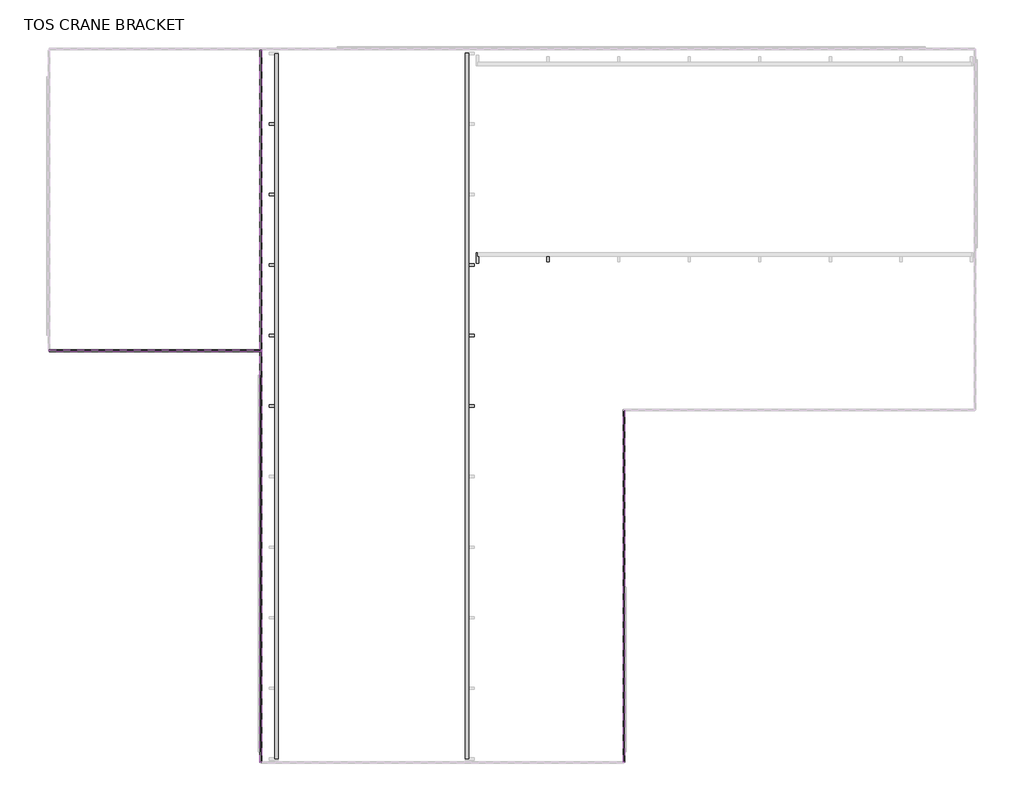
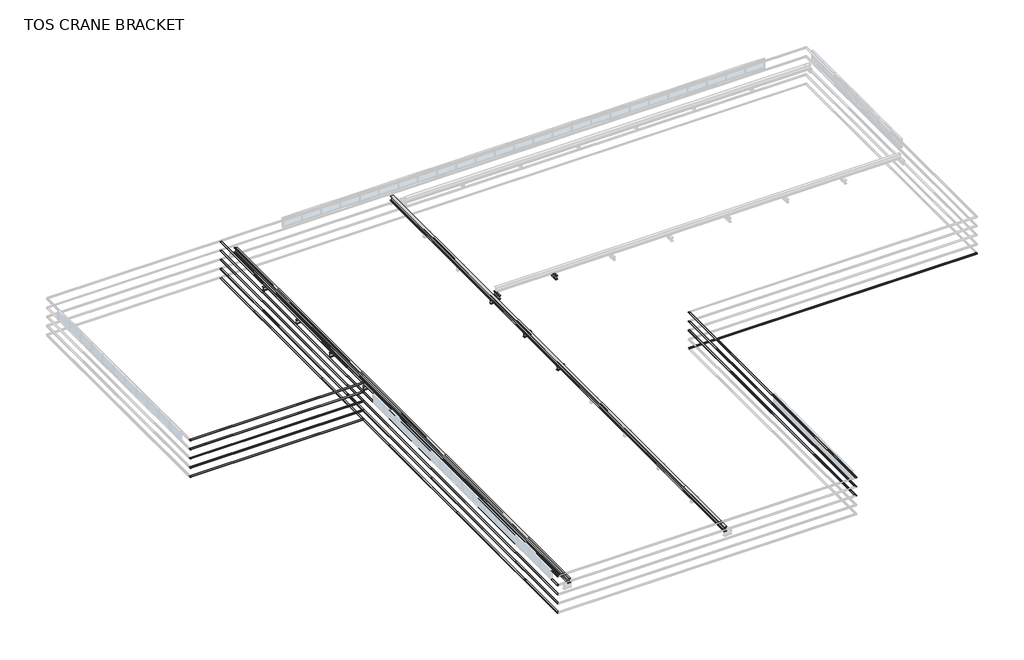
# One storey, part 2 of 3: 26 beams.
"""IFC4 building model written with IfcOpenShell, lengths in millimetres."""

import ifcopenshell
import ifcopenshell.guid

model = None  # the IFC model being written
_history = None  # IfcOwnerHistory: only IFC2X3 demands one
_inside = {}  # id of a spatial element -> (the spatial element, [elements in it])
_under = {}  # id of a project, library or spatial element -> (it, [spatial elements below it])
_declared = {}  # id of a project -> (the project, [libraries it declares])
_typed = {}  # id of a type object -> (the type object, [elements of that type])
_made_of = {}  # id of a material, layer set ... -> (it, [elements and type objects made of it])


def new_model(schema):
    """Start an empty IFC model of exactly this schema.

    Asked for "IFC4X3", IfcOpenShell would pick the latest addendum, in which some entities
    have other attributes; the version numbers below select the first issue.
    IFC2X3 requires an IfcOwnerHistory on every rooted entity: one is made here for all.
    """
    global model, _history
    if schema == "IFC4X3":
        model = ifcopenshell.file(schema_version=(4, 3, 0, 0))
    else:
        model = ifcopenshell.file(schema=schema)
    _inside.clear()
    _under.clear()
    _declared.clear()
    _typed.clear()
    _made_of.clear()
    _history = None
    if model.schema == "IFC2X3":
        org = make("IfcOrganization", Name="unknown")
        user = make(
            "IfcPersonAndOrganization",
            ThePerson=make("IfcPerson", FamilyName="unknown"),
            TheOrganization=org,
        )
        app = make(
            "IfcApplication",
            ApplicationDeveloper=org,
            Version="unknown",
            ApplicationFullName="unknown",
            ApplicationIdentifier="unknown",
        )
        _history = make(
            "IfcOwnerHistory",
            OwningUser=user,
            OwningApplication=app,
            ChangeAction="ADDED",
            CreationDate=0,
        )
    return model


def make(cls, **values):
    """One entity of the class cls with the attributes given. An attribute that is None is left unset."""
    return model.create_entity(
        cls, **{name: value for name, value in values.items() if value is not None}
    )


def rooted(cls, **values):
    """An entity with a GlobalId (a new one), such as an element, a storey or a relation."""
    return make(cls, GlobalId=ifcopenshell.guid.new(), OwnerHistory=_history, **values)


def si_unit(unit_type, name, prefix=None):
    """IfcSIUnit, for example si_unit("LENGTHUNIT", "METRE", prefix="MILLI")."""
    return make("IfcSIUnit", UnitType=unit_type, Prefix=prefix, Name=name)


def assignment(units):
    """IfcUnitAssignment: the units of a project."""
    return None if units is None else make("IfcUnitAssignment", Units=units)


def point(xyz):
    """IfcCartesianPoint."""
    return None if xyz is None else make("IfcCartesianPoint", Coordinates=xyz)


def direction(xyz):
    """IfcDirection."""
    return None if xyz is None else make("IfcDirection", DirectionRatios=xyz)


def frame(location, z_axis=None, x_axis=None):
    """IfcAxis2Placement3D, a coordinate frame: its origin and axes. An axis left out is left unset."""
    return make(
        "IfcAxis2Placement3D",
        Location=point(location),
        Axis=direction(z_axis),
        RefDirection=direction(x_axis),
    )


def frame_2d(location, x_axis=None):
    """IfcAxis2Placement2D, a coordinate frame in the plane: its origin and x axis."""
    return make(
        "IfcAxis2Placement2D", Location=point(location), RefDirection=direction(x_axis)
    )


def origin():
    """The frame at (0, 0, 0) with its axes left unset."""
    return frame((0.0, 0.0, 0.0))


def place(relative_to, where):
    """IfcLocalPlacement: puts the frame where relative to a parent placement (None: the world)."""
    return make(
        "IfcLocalPlacement", PlacementRelTo=relative_to, RelativePlacement=where
    )


def context(
    kind, dimensions, precision=None, world=None, true_north=None, identifier=None
):
    """IfcGeometricRepresentationContext, for example the 3D "Model" context."""
    return make(
        "IfcGeometricRepresentationContext",
        ContextIdentifier=identifier,
        ContextType=kind,
        CoordinateSpaceDimension=dimensions,
        Precision=precision,
        WorldCoordinateSystem=world,
        TrueNorth=true_north,
    )


def project(units=None, contexts=None):
    """IfcProject with its units and contexts."""
    return rooted(
        "IfcProject",
        Name="project",
        RepresentationContexts=contexts,
        UnitsInContext=assignment(units),
    )


def spatial(cls, under=None, at=None, **own):
    """A site, building, storey or space (cls), placed at a placement, below another one or the project."""
    s = rooted(cls, ObjectPlacement=at, **own)
    if under is not None:
        _under.setdefault(under.id(), (under, []))[1].append(s)
    return s


def polyline(points):
    """IfcPolyline through the points."""
    return make("IfcPolyline", Points=[point(p) for p in points])


def circle_curve(where, radius):
    """IfcCircle in the frame where."""
    return make("IfcCircle", Position=where, Radius=radius)


def trimmed(basis, trim1, trim2, sense, master):
    """IfcTrimmedCurve: the piece of a basis curve between two trims."""
    return make(
        "IfcTrimmedCurve",
        BasisCurve=basis,
        Trim1=trim1,
        Trim2=trim2,
        SenseAgreement=sense,
        MasterRepresentation=master,
    )


def segment(curve, same_sense, transition):
    """IfcCompositeCurveSegment."""
    return make(
        "IfcCompositeCurveSegment",
        Transition=transition,
        SameSense=same_sense,
        ParentCurve=curve,
    )


def composite_curve(segments, self_intersect=None):
    """IfcCompositeCurve: segments joined end to end."""
    return make("IfcCompositeCurve", Segments=segments, SelfIntersect=self_intersect)


def outline(outer, holes=None, kind="AREA"):
    """IfcArbitraryClosedProfileDef: a profile drawn as a closed curve; with holes, ...WithVoids."""
    if holes is None:
        return make("IfcArbitraryClosedProfileDef", ProfileType=kind, OuterCurve=outer)
    return make(
        "IfcArbitraryProfileDefWithVoids",
        ProfileType=kind,
        OuterCurve=outer,
        InnerCurves=holes,
    )


def extrude(swept, where, along, depth):
    """IfcExtrudedAreaSolid: the profile swept, set in the frame where, extruded along a direction by depth."""
    return make(
        "IfcExtrudedAreaSolid",
        SweptArea=swept,
        Position=where,
        ExtrudedDirection=direction(along),
        Depth=depth,
    )


def shape(context_of_items, identifier, shape_type, items):
    """IfcShapeRepresentation: the items that make up one representation, for example the "Body"."""
    return make(
        "IfcShapeRepresentation",
        ContextOfItems=context_of_items,
        RepresentationIdentifier=identifier,
        RepresentationType=shape_type,
        Items=items,
    )


def source(mapping_origin, context_of_items, identifier, shape_type, items):
    """IfcRepresentationMap: a shape defined once, which mapped items show again and again."""
    return make(
        "IfcRepresentationMap",
        MappingOrigin=mapping_origin,
        MappedRepresentation=shape(context_of_items, identifier, shape_type, items),
    )


def transform(
    local_origin,
    x_axis=None,
    y_axis=None,
    z_axis=None,
    scale=None,
    scale2=None,
    scale3=None,
    uniform=True,
):
    """IfcCartesianTransformationOperator3D, or its non-uniform kind. x_axis, y_axis, z_axis: its Axis1, 2, 3."""
    if uniform:
        return make(
            "IfcCartesianTransformationOperator3D",
            Axis1=direction(x_axis),
            Axis2=direction(y_axis),
            LocalOrigin=point(local_origin),
            Scale=scale,
            Axis3=direction(z_axis),
        )
    return make(
        "IfcCartesianTransformationOperator3DnonUniform",
        Axis1=direction(x_axis),
        Axis2=direction(y_axis),
        LocalOrigin=point(local_origin),
        Scale=scale,
        Axis3=direction(z_axis),
        Scale2=scale2,
        Scale3=scale3,
    )


def mapped(mapping_source, mapping_target):
    """IfcMappedItem: shows the shape of a source again, moved by a transform."""
    return make(
        "IfcMappedItem", MappingSource=mapping_source, MappingTarget=mapping_target
    )


def made_of(thing, what):
    """Note that an element or type object is made of a material, layer set ...; save() writes the relation."""
    if what is not None:
        _made_of.setdefault(what.id(), (what, []))[1].append(thing)
    return thing


def element(
    cls,
    number,
    at=None,
    inside=None,
    cuts=None,
    type_object=None,
    material=None,
    context=None,
    identifier="Body",
    shape_type=None,
    held_by="IfcProductDefinitionShape",
    body=None,
    shapes=None,
    **own,
):
    """One element of the class cls, such as IfcWall. Its Tag is "e" and its number.

    at: its placement. inside: the storey or other place that contains it. cuts: it is an
    opening in that element (IfcRelVoidsElement). A single representation is given by context,
    identifier, shape_type and body (its items); several are given by shapes. held_by: the class
    of the entity that holds the representations. save() writes the other relations.
    """
    e = rooted(cls, Tag="e%d" % number, ObjectPlacement=at, **own)
    if body is not None:
        shapes = [shape(context, identifier, shape_type, body)]
    if shapes is not None:
        e.Representation = make(held_by, Representations=shapes)
    if inside is not None:
        _inside.setdefault(inside.id(), (inside, []))[1].append(e)
    if cuts is not None:
        rooted(
            "IfcRelVoidsElement", RelatingBuildingElement=cuts, RelatedOpeningElement=e
        )
    if type_object is not None:
        _typed.setdefault(type_object.id(), (type_object, []))[1].append(e)
    return made_of(e, material)


def aggregate(whole, parts):
    """IfcRelAggregates: a whole, such as a stair, and the parts it consists of."""
    return rooted("IfcRelAggregates", RelatingObject=whole, RelatedObjects=parts)


def save(model, path):
    """Write the relations noted so far, then the file.

    IfcRelAggregates (storeys below a building ...), IfcRelContainedInSpatialStructure (elements
    in a storey), IfcRelDefinesByType, IfcRelAssociatesMaterial and IfcRelDeclares: one each for
    every whole, place, type object, material and project.
    """
    for whole, parts in _under.values():
        aggregate(whole, parts)
    for where, things in _inside.values():
        rooted(
            "IfcRelContainedInSpatialStructure",
            RelatedElements=things,
            RelatingStructure=where,
        )
    for kind, things in _typed.values():
        rooted("IfcRelDefinesByType", RelatedObjects=things, RelatingType=kind)
    for what, things in _made_of.values():
        rooted("IfcRelAssociatesMaterial", RelatedObjects=things, RelatingMaterial=what)
    for by, libraries in _declared.values():
        rooted("IfcRelDeclares", RelatingContext=by, RelatedDefinitions=libraries)
    model.write(path)


def beam_70e5a2de(model_context):
    return source(origin(), model_context, "Body", "SweptSolid", [
        extrude(outline(composite_curve([segment(polyline([(150.0, -226.0), (150.0, -244.0), (-150.0, -244.0), (-150.0, -226.0), (-31.5, -226.0)]), True, "CONTINUOUS"), segment(trimmed(circle_curve(frame_2d((-31.5, -200.0)), 26.0), [point((-31.5, -226.0))], [point((-5.5, -200.0))], True, "CARTESIAN"), True, "CONTINUOUS"), segment(polyline([(-5.5, -200.0), (-5.5, 200.0)]), True, "CONTINUOUS"), segment(trimmed(circle_curve(frame_2d((-31.5, 200.0)), 26.0), [point((-5.5, 200.0))], [point((-31.5, 226.0))], True, "CARTESIAN"), True, "CONTINUOUS"), segment(polyline([(-31.5, 226.0), (-150.0, 226.0), (-150.0, 244.0), (150.0, 244.0), (150.0, 226.0), (31.5, 226.0)]), True, "CONTINUOUS"), segment(trimmed(circle_curve(frame_2d((31.5, 200.0)), 26.0), [point((31.5, 226.0))], [point((5.5, 200.0))], True, "CARTESIAN"), True, "CONTINUOUS"), segment(polyline([(5.5, 200.0), (5.5, -200.0)]), True, "CONTINUOUS"), segment(trimmed(circle_curve(frame_2d((31.5, -200.0)), 26.0), [point((5.5, -200.0))], [point((31.5, -226.0))], True, "CARTESIAN"), True, "CONTINUOUS"), segment(polyline([(31.5, -226.0), (150.0, -226.0)]), True, "CONTINUOUS")], self_intersect=False)), frame((-30000.0, 0.0, 0.0), z_axis=(1.0, 0.0, 0.0), x_axis=(0.0, 1.0, 0.0)), (0.0, 0.0, 1.0), 60000.0),
    ])


def beam_a081c7c9(model_context):
    return source(origin(), model_context, "Body", "SweptSolid", [
        extrude(outline(composite_curve([segment(polyline([(100.0, -187.0), (100.0, -200.0), (-100.0, -200.0), (-100.0, -187.0), (-20.0, -187.0)]), True, "CONTINUOUS"), segment(trimmed(circle_curve(frame_2d((-20.0, -171.0)), 16.0), [point((-20.0, -187.0))], [point((-4.0, -171.0))], True, "CARTESIAN"), True, "CONTINUOUS"), segment(polyline([(-4.0, -171.0), (-4.0, 171.0)]), True, "CONTINUOUS"), segment(trimmed(circle_curve(frame_2d((-20.0, 171.0)), 16.0), [point((-4.0, 171.0))], [point((-20.0, 187.0))], True, "CARTESIAN"), True, "CONTINUOUS"), segment(polyline([(-20.0, 187.0), (-100.0, 187.0), (-100.0, 200.0), (100.0, 200.0), (100.0, 187.0), (20.0, 187.0)]), True, "CONTINUOUS"), segment(trimmed(circle_curve(frame_2d((20.0, 171.0)), 16.0), [point((20.0, 187.0))], [point((4.0, 171.0))], True, "CARTESIAN"), True, "CONTINUOUS"), segment(polyline([(4.0, 171.0), (4.0, -171.0)]), True, "CONTINUOUS"), segment(trimmed(circle_curve(frame_2d((20.0, -171.0)), 16.0), [point((4.0, -171.0))], [point((20.0, -187.0))], True, "CARTESIAN"), True, "CONTINUOUS"), segment(polyline([(20.0, -187.0), (100.0, -187.0)]), True, "CONTINUOUS")], self_intersect=False)), frame((-236.0, 0.0, 0.0), z_axis=(1.0, 0.0, 0.0), x_axis=(0.0, 1.0, 0.0)), (0.0, 0.0, 1.0), 766.0),
    ])


def beam_d36fe593(model_context):
    return source(origin(), model_context, "Body", "SweptSolid", [
        extrude(outline(composite_curve([segment(polyline([(-100.0, -187.0), (-20.0, -187.0)]), True, "CONTINUOUS"), segment(trimmed(circle_curve(frame_2d((-20.0, -171.0)), 16.0), [point((-20.0, -187.0))], [point((-4.0, -171.0))], True, "CARTESIAN"), True, "CONTINUOUS"), segment(polyline([(-4.0, -171.0), (-4.0, 171.0)]), True, "CONTINUOUS"), segment(trimmed(circle_curve(frame_2d((-20.0, 171.0)), 16.0), [point((-4.0, 171.0))], [point((-20.0, 187.0))], True, "CARTESIAN"), True, "CONTINUOUS"), segment(polyline([(-20.0, 187.0), (-100.0, 187.0), (-100.0, 200.0), (100.0, 200.0), (100.0, 187.0), (20.0, 187.0)]), True, "CONTINUOUS"), segment(trimmed(circle_curve(frame_2d((20.0, 171.0)), 16.0), [point((20.0, 187.0))], [point((4.0, 171.0))], True, "CARTESIAN"), True, "CONTINUOUS"), segment(polyline([(4.0, 171.0), (4.0, -171.0)]), True, "CONTINUOUS"), segment(trimmed(circle_curve(frame_2d((20.0, -171.0)), 16.0), [point((4.0, -171.0))], [point((20.0, -187.0))], True, "CARTESIAN"), True, "CONTINUOUS"), segment(polyline([(20.0, -187.0), (100.0, -187.0), (100.0, -200.0), (-100.0, -200.0), (-100.0, -187.0)]), True, "CONTINUOUS")], self_intersect=False)), frame((-236.0, 0.0, 0.0), z_axis=(1.0, 0.0, 0.0), x_axis=(0.0, 1.0, 0.0)), (0.0, 0.0, 1.0), 766.0),
    ])


def beam_06871935(model_context):
    return source(origin(), model_context, "Body", "SweptSolid", [
        extrude(outline(composite_curve([segment(polyline([(-150.0, -226.0), (-31.5, -226.0)]), True, "CONTINUOUS"), segment(trimmed(circle_curve(frame_2d((-31.5, -200.0)), 26.0), [point((-31.5, -226.0))], [point((-5.5, -200.0))], True, "CARTESIAN"), True, "CONTINUOUS"), segment(polyline([(-5.5, -200.0), (-5.5, 200.0)]), True, "CONTINUOUS"), segment(trimmed(circle_curve(frame_2d((-31.5, 200.0)), 26.0), [point((-5.5, 200.0))], [point((-31.5, 226.0))], True, "CARTESIAN"), True, "CONTINUOUS"), segment(polyline([(-31.5, 226.0), (-150.0, 226.0), (-150.0, 244.0), (150.0, 244.0), (150.0, 226.0), (31.5, 226.0)]), True, "CONTINUOUS"), segment(trimmed(circle_curve(frame_2d((31.5, 200.0)), 26.0), [point((31.5, 226.0))], [point((5.5, 200.0))], True, "CARTESIAN"), True, "CONTINUOUS"), segment(polyline([(5.5, 200.0), (5.5, -200.0)]), True, "CONTINUOUS"), segment(trimmed(circle_curve(frame_2d((31.5, -200.0)), 26.0), [point((5.5, -200.0))], [point((31.5, -226.0))], True, "CARTESIAN"), True, "CONTINUOUS"), segment(polyline([(31.5, -226.0), (150.0, -226.0), (150.0, -244.0), (-150.0, -244.0), (-150.0, -226.0)]), True, "CONTINUOUS")], self_intersect=False)), frame((-29987.2, 0.0, 0.0), z_axis=(1.0, 0.0, 0.0), x_axis=(0.0, 1.0, 0.0)), (0.0, 0.0, 1.0), 59974.4),
    ])


def beam_29f4eb64(model_context):
    return source(origin(), model_context, "Body", "SweptSolid", [
        extrude(outline(composite_curve([segment(polyline([(-100.0, -187.0), (-20.0, -187.0)]), True, "CONTINUOUS"), segment(trimmed(circle_curve(frame_2d((-20.0, -171.0)), 16.0), [point((-20.0, -187.0))], [point((-4.0, -171.0))], True, "CARTESIAN"), True, "CONTINUOUS"), segment(polyline([(-4.0, -171.0), (-4.0, 171.0)]), True, "CONTINUOUS"), segment(trimmed(circle_curve(frame_2d((-20.0, 171.0)), 16.0), [point((-4.0, 171.0))], [point((-20.0, 187.0))], True, "CARTESIAN"), True, "CONTINUOUS"), segment(polyline([(-20.0, 187.0), (-100.0, 187.0), (-100.0, 200.0), (100.0, 200.0), (100.0, 187.0), (20.0, 187.0)]), True, "CONTINUOUS"), segment(trimmed(circle_curve(frame_2d((20.0, 171.0)), 16.0), [point((20.0, 187.0))], [point((4.0, 171.0))], True, "CARTESIAN"), True, "CONTINUOUS"), segment(polyline([(4.0, 171.0), (4.0, -171.0)]), True, "CONTINUOUS"), segment(trimmed(circle_curve(frame_2d((20.0, -171.0)), 16.0), [point((4.0, -171.0))], [point((20.0, -187.0))], True, "CARTESIAN"), True, "CONTINUOUS"), segment(polyline([(20.0, -187.0), (100.0, -187.0), (100.0, -200.0), (-100.0, -200.0), (-100.0, -187.0)]), True, "CONTINUOUS")], self_intersect=False)), frame((-380.0, 0.0, 0.0), z_axis=(1.0, 0.0, 0.0), x_axis=(0.0, 1.0, 0.0)), (0.0, 0.0, 1.0), 910.0),
    ])


def steel_framing_lc_58cf0942(model_context):
    return source(origin(), model_context, "Body", "SweptSolid", [
        extrude(outline(composite_curve([segment(polyline([(18.6, 67.0), (18.6, -67.0)]), True, "CONTINUOUS"), segment(trimmed(circle_curve(frame_2d((10.6, -67.0)), 8.0), [point((18.6, -67.0))], [point((10.6, -75.0))], False, "CARTESIAN"), True, "CONTINUOUS"), segment(polyline([(10.6, -75.0), (-48.4, -75.0)]), True, "CONTINUOUS"), segment(trimmed(circle_curve(frame_2d((-48.4, -67.0)), 8.0), [point((-48.4, -75.0))], [point((-56.4, -67.0))], False, "CARTESIAN"), True, "CONTINUOUS"), segment(polyline([(-56.4, -67.0), (-56.4, -50.0), (-53.2, -50.0), (-53.2, -67.0)]), True, "CONTINUOUS"), segment(trimmed(circle_curve(frame_2d((-48.4, -67.0)), 4.8), [point((-53.2, -67.0))], [point((-48.4, -71.8))], True, "CARTESIAN"), True, "CONTINUOUS"), segment(polyline([(-48.4, -71.8), (10.6, -71.8)]), True, "CONTINUOUS"), segment(trimmed(circle_curve(frame_2d((10.6, -67.0)), 4.8), [point((10.6, -71.8))], [point((15.4, -67.0))], True, "CARTESIAN"), True, "CONTINUOUS"), segment(polyline([(15.4, -67.0), (15.4, 67.0)]), True, "CONTINUOUS"), segment(trimmed(circle_curve(frame_2d((10.6, 67.0)), 4.8), [point((15.4, 67.0))], [point((10.6, 71.8))], True, "CARTESIAN"), True, "CONTINUOUS"), segment(polyline([(10.6, 71.8), (-48.4, 71.8)]), True, "CONTINUOUS"), segment(trimmed(circle_curve(frame_2d((-48.4, 67.0)), 4.8), [point((-48.4, 71.8))], [point((-53.2, 67.0))], True, "CARTESIAN"), True, "CONTINUOUS"), segment(polyline([(-53.2, 67.0), (-53.2, 50.0), (-56.4, 50.0), (-56.4, 67.0)]), True, "CONTINUOUS"), segment(trimmed(circle_curve(frame_2d((-48.4, 67.0)), 8.0), [point((-56.4, 67.0))], [point((-48.4, 75.0))], False, "CARTESIAN"), True, "CONTINUOUS"), segment(polyline([(-48.4, 75.0), (10.6, 75.0)]), True, "CONTINUOUS"), segment(trimmed(circle_curve(frame_2d((10.6, 67.0)), 8.0), [point((10.6, 75.0))], [point((18.6, 67.0))], False, "CARTESIAN"), True, "CONTINUOUS")], self_intersect=False)), frame((-30297.0, 0.0, 0.0), z_axis=(1.0, 0.0, 0.0), x_axis=(0.0, 1.0, 0.0)), (0.0, 0.0, 1.0), 60581.0),
    ])


model = new_model("IFC4")

# Units and contexts
model_context = context("Model", 3, world=origin())
ifc_project = project(units=[si_unit("LENGTHUNIT", "METRE", prefix="MILLI")], contexts=[model_context])

# Site, building, storey
site = spatial("IfcSite", under=ifc_project)
building = spatial("IfcBuilding", under=site)
storey = spatial("IfcBuildingStorey", under=building, Name="TOS CRANE BRACKET", Elevation=6699.9618634)

# Beams
placement = place(None, origin())
beam_shape = beam_70e5a2de(model_context)
element("IfcBeam", 1, ObjectType="Steel Framing_H_KS : H_SB_AR_S02_H-488x300x11x18_CRG1", at=placement, inside=storey, context=model_context, shape_type="MappedRepresentation", body=[
    mapped(beam_shape, transform((35100.0, -30000.0, 6953.9618634), x_axis=(0.0, 1.0, 0.0), y_axis=(-1.0, 0.0, 0.0), z_axis=(0.0, 0.0, 1.0))),
])
beam_2_shape = beam_a081c7c9(model_context)
element("IfcBeam", 2, ObjectType="Steel Framing_H_KS : H_SB_AR_S02_H-400x200x8x13_SCB1", at=placement, inside=storey, context=model_context, shape_type="MappedRepresentation", body=[
    mapped(beam_2_shape, transform((35470.0, -18000.0, 6499.9618634), x_axis=(-1.0, 0.0, 0.0), y_axis=(0.0, -1.0, 0.0), z_axis=(0.0, 0.0, 1.0))),
])
element("IfcBeam", 3, ObjectType="Steel Framing_H_KS : H_SB_AR_S02_H-400x200x8x13_SCB1", at=placement, inside=storey, context=model_context, shape_type="MappedRepresentation", body=[
    mapped(beam_2_shape, transform((35470.0, -24000.0, 6499.9618634), x_axis=(-1.0, 0.0, 0.0), y_axis=(0.0, -1.0, 0.0), z_axis=(0.0, 0.0, 1.0))),
])
element("IfcBeam", 4, ObjectType="Steel Framing_H_KS : H_SB_AR_S02_H-400x200x8x13_SCB1", at=placement, inside=storey, context=model_context, shape_type="MappedRepresentation", body=[
    mapped(beam_2_shape, transform((35470.0, -30000.0, 6499.9618634), x_axis=(-1.0, 0.0, 0.0), y_axis=(0.0, -1.0, 0.0), z_axis=(0.0, 0.0, 1.0))),
])
beam_3_shape = beam_d36fe593(model_context)
element("IfcBeam", 5, ObjectType="Steel Framing_H_KS : H_SB_AR_S02_H-400x200x8x13_SCB1", at=placement, inside=storey, context=model_context, shape_type="MappedRepresentation", body=[
    mapped(beam_3_shape, transform((18530.0, -6000.0, 6499.9618634), x_axis=(1.0, 0.0, 0.0), y_axis=(0.0, 1.0, 0.0), z_axis=(0.0, 0.0, 1.0))),
])
element("IfcBeam", 6, ObjectType="Steel Framing_H_KS : H_SB_AR_S02_H-400x200x8x13_SCB1", at=placement, inside=storey, context=model_context, shape_type="MappedRepresentation", body=[
    mapped(beam_3_shape, transform((18530.0, -12000.0, 6499.9618634), x_axis=(1.0, 0.0, 0.0), y_axis=(0.0, 1.0, 0.0), z_axis=(0.0, 0.0, 1.0))),
])
element("IfcBeam", 7, ObjectType="Steel Framing_H_KS : H_SB_AR_S02_H-400x200x8x13_SCB1", at=placement, inside=storey, context=model_context, shape_type="MappedRepresentation", body=[
    mapped(beam_3_shape, transform((18530.0, -18000.0, 6499.9618634), x_axis=(1.0, 0.0, 0.0), y_axis=(0.0, 1.0, 0.0), z_axis=(0.0, 0.0, 1.0))),
])
element("IfcBeam", 8, ObjectType="Steel Framing_H_KS : H_SB_AR_S02_H-400x200x8x13_SCB1", at=placement, inside=storey, context=model_context, shape_type="MappedRepresentation", body=[
    mapped(beam_3_shape, transform((18530.0, -24000.0, 6499.9618634), x_axis=(1.0, 0.0, 0.0), y_axis=(0.0, 1.0, 0.0), z_axis=(0.0, 0.0, 1.0))),
])
element("IfcBeam", 9, ObjectType="Steel Framing_H_KS : H_SB_AR_S02_H-400x200x8x13_SCB1", at=placement, inside=storey, context=model_context, shape_type="MappedRepresentation", body=[
    mapped(beam_3_shape, transform((18530.0, -30000.0, 6499.9618634), x_axis=(1.0, 0.0, 0.0), y_axis=(0.0, 1.0, 0.0), z_axis=(0.0, 0.0, 1.0))),
])
element("IfcBeam", 10, ObjectType="Steel Framing_H_KS : H_SB_AR_S02_H-400x200x8x13_SCB1", at=placement, inside=storey, context=model_context, shape_type="MappedRepresentation", body=[
    mapped(beam_3_shape, transform((42000.0, -17470.0, 6499.9618634), x_axis=(0.0, 1.0, 0.0), y_axis=(-1.0, 0.0, 0.0), z_axis=(0.0, 0.0, 1.0))),
])
beam_4_shape = beam_06871935(model_context)
element("IfcBeam", 11, ObjectType="Steel Framing_H_KS : H_SB_AR_S02_H-488x300x11x18_CRG1", at=placement, inside=storey, context=model_context, shape_type="MappedRepresentation", body=[
    mapped(beam_4_shape, transform((18900.0, -30000.0, 6953.9618634), x_axis=(0.0, 1.0, 0.0), y_axis=(-1.0, 0.0, 0.0), z_axis=(0.0, 0.0, 1.0))),
])
beam_5_shape = beam_29f4eb64(model_context)
element("IfcBeam", 12, ObjectType="Steel Framing_H_KS : H_SB_AR_S02_H-400x200x8x13_SCB1", at=placement, inside=storey, context=model_context, shape_type="MappedRepresentation", body=[
    mapped(beam_5_shape, transform((36000.0, -17470.0, 6499.9618634), x_axis=(0.0, 1.0, 0.0), y_axis=(-1.0, 0.0, 0.0), z_axis=(0.0, 0.0, 1.0))),
])
element("IfcBeam", 13, ObjectType="Steel Framing_LC : H_SB_AR_S00_LC-150x75x25x3.2", at=placement, inside=storey, context=model_context, shape_type="SweptSolid", body=[
    extrude(outline(composite_curve([segment(trimmed(circle_curve(frame_2d((-25233.0, 4160.5618634)), 8.0), [point((-25233.0, 4168.5618634))], [point((-25225.0, 4160.5618634))], False, "CARTESIAN"), True, "CONTINUOUS"), segment(polyline([(-25225.0, 4160.5618634), (-25225.0, 4101.5618634)]), True, "CONTINUOUS"), segment(trimmed(circle_curve(frame_2d((-25233.0, 4101.5618634)), 8.0), [point((-25225.0, 4101.5618634))], [point((-25233.0, 4093.5618634))], False, "CARTESIAN"), True, "CONTINUOUS"), segment(polyline([(-25233.0, 4093.5618634), (-25250.0, 4093.5618634), (-25250.0, 4096.7618634), (-25233.0, 4096.7618634)]), True, "CONTINUOUS"), segment(trimmed(circle_curve(frame_2d((-25233.0, 4101.5618634)), 4.8), [point((-25233.0, 4096.7618634))], [point((-25228.2, 4101.5618634))], True, "CARTESIAN"), True, "CONTINUOUS"), segment(polyline([(-25228.2, 4101.5618634), (-25228.2, 4160.5618634)]), True, "CONTINUOUS"), segment(trimmed(circle_curve(frame_2d((-25233.0, 4160.5618634)), 4.8), [point((-25228.2, 4160.5618634))], [point((-25233.0, 4165.3618634))], True, "CARTESIAN"), True, "CONTINUOUS"), segment(polyline([(-25233.0, 4165.3618634), (-25367.0, 4165.3618634)]), True, "CONTINUOUS"), segment(trimmed(circle_curve(frame_2d((-25367.0, 4160.5618634)), 4.8), [point((-25367.0, 4165.3618634))], [point((-25371.8, 4160.5618634))], True, "CARTESIAN"), True, "CONTINUOUS"), segment(polyline([(-25371.8, 4160.5618634), (-25371.8, 4101.5618634)]), True, "CONTINUOUS"), segment(trimmed(circle_curve(frame_2d((-25367.0, 4101.5618634)), 4.8), [point((-25371.8, 4101.5618634))], [point((-25367.0, 4096.7618634))], True, "CARTESIAN"), True, "CONTINUOUS"), segment(polyline([(-25367.0, 4096.7618634), (-25350.0, 4096.7618634), (-25350.0, 4093.5618634), (-25367.0, 4093.5618634)]), True, "CONTINUOUS"), segment(trimmed(circle_curve(frame_2d((-25367.0, 4101.5618634)), 8.0), [point((-25367.0, 4093.5618634))], [point((-25375.0, 4101.5618634))], False, "CARTESIAN"), True, "CONTINUOUS"), segment(polyline([(-25375.0, 4101.5618634), (-25375.0, 4160.5618634)]), True, "CONTINUOUS"), segment(trimmed(circle_curve(frame_2d((-25367.0, 4160.5618634)), 8.0), [point((-25375.0, 4160.5618634))], [point((-25367.0, 4168.5618634))], False, "CARTESIAN"), True, "CONTINUOUS"), segment(polyline([(-25367.0, 4168.5618634), (-25233.0, 4168.5618634)]), True, "CONTINUOUS")], self_intersect=False)), frame((-450.0, 0.0, 0.0), z_axis=(1.0, 0.0, 0.0), x_axis=(0.0, 1.0, 0.0)), (0.0, 0.0, 1.0), 18000.0),
])
element("IfcBeam", 14, ObjectType="Steel Framing_LC : H_SB_AR_S00_LC-150x75x25x3.2", at=placement, inside=storey, context=model_context, shape_type="SweptSolid", body=[
    extrude(outline(composite_curve([segment(polyline([(-30392.0, 4168.5618634), (-30258.0, 4168.5618634)]), True, "CONTINUOUS"), segment(trimmed(circle_curve(frame_2d((-30258.0, 4160.5618634)), 8.0), [point((-30258.0, 4168.5618634))], [point((-30250.0, 4160.5618634))], False, "CARTESIAN"), True, "CONTINUOUS"), segment(polyline([(-30250.0, 4160.5618634), (-30250.0, 4101.5618634)]), True, "CONTINUOUS"), segment(trimmed(circle_curve(frame_2d((-30258.0, 4101.5618634)), 8.0), [point((-30250.0, 4101.5618634))], [point((-30258.0, 4093.5618634))], False, "CARTESIAN"), True, "CONTINUOUS"), segment(polyline([(-30258.0, 4093.5618634), (-30275.0, 4093.5618634), (-30275.0, 4096.7618634), (-30258.0, 4096.7618634)]), True, "CONTINUOUS"), segment(trimmed(circle_curve(frame_2d((-30258.0, 4101.5618634)), 4.8), [point((-30258.0, 4096.7618634))], [point((-30253.2, 4101.5618634))], True, "CARTESIAN"), True, "CONTINUOUS"), segment(polyline([(-30253.2, 4101.5618634), (-30253.2, 4160.5618634)]), True, "CONTINUOUS"), segment(trimmed(circle_curve(frame_2d((-30258.0, 4160.5618634)), 4.8), [point((-30253.2, 4160.5618634))], [point((-30258.0, 4165.3618634))], True, "CARTESIAN"), True, "CONTINUOUS"), segment(polyline([(-30258.0, 4165.3618634), (-30392.0, 4165.3618634)]), True, "CONTINUOUS"), segment(trimmed(circle_curve(frame_2d((-30392.0, 4160.5618634)), 4.8), [point((-30392.0, 4165.3618634))], [point((-30396.8, 4160.5618634))], True, "CARTESIAN"), True, "CONTINUOUS"), segment(polyline([(-30396.8, 4160.5618634), (-30396.8, 4101.5618634)]), True, "CONTINUOUS"), segment(trimmed(circle_curve(frame_2d((-30392.0, 4101.5618634)), 4.8), [point((-30396.8, 4101.5618634))], [point((-30392.0, 4096.7618634))], True, "CARTESIAN"), True, "CONTINUOUS"), segment(polyline([(-30392.0, 4096.7618634), (-30375.0, 4096.7618634), (-30375.0, 4093.5618634), (-30392.0, 4093.5618634)]), True, "CONTINUOUS"), segment(trimmed(circle_curve(frame_2d((-30392.0, 4101.5618634)), 8.0), [point((-30392.0, 4093.5618634))], [point((-30400.0, 4101.5618634))], False, "CARTESIAN"), True, "CONTINUOUS"), segment(polyline([(-30400.0, 4101.5618634), (-30400.0, 4160.5618634)]), True, "CONTINUOUS"), segment(trimmed(circle_curve(frame_2d((-30392.0, 4160.5618634)), 8.0), [point((-30400.0, 4160.5618634))], [point((-30392.0, 4168.5618634))], False, "CARTESIAN"), True, "CONTINUOUS")], self_intersect=False)), frame((48450.0, 0.0, 0.0), z_axis=(1.0, 0.0, 0.0), x_axis=(0.0, 1.0, 0.0)), (0.0, 0.0, 1.0), 29850.0),
])
element("IfcBeam", 15, ObjectType="Steel Framing_LC : H_SB_AR_S00_LC-150x75x25x3.2", at=placement, inside=storey, context=model_context, shape_type="SweptSolid", body=[
    extrude(outline(composite_curve([segment(trimmed(circle_curve(frame_2d((-25233.0, 5160.5618634)), 8.0), [point((-25233.0, 5168.5618634))], [point((-25225.0, 5160.5618634))], False, "CARTESIAN"), True, "CONTINUOUS"), segment(polyline([(-25225.0, 5160.5618634), (-25225.0, 5101.5618634)]), True, "CONTINUOUS"), segment(trimmed(circle_curve(frame_2d((-25233.0, 5101.5618634)), 8.0), [point((-25225.0, 5101.5618634))], [point((-25233.0, 5093.5618634))], False, "CARTESIAN"), True, "CONTINUOUS"), segment(polyline([(-25233.0, 5093.5618634), (-25250.0, 5093.5618634), (-25250.0, 5096.7618634), (-25233.0, 5096.7618634)]), True, "CONTINUOUS"), segment(trimmed(circle_curve(frame_2d((-25233.0, 5101.5618634)), 4.8), [point((-25233.0, 5096.7618634))], [point((-25228.2, 5101.5618634))], True, "CARTESIAN"), True, "CONTINUOUS"), segment(polyline([(-25228.2, 5101.5618634), (-25228.2, 5160.5618634)]), True, "CONTINUOUS"), segment(trimmed(circle_curve(frame_2d((-25233.0, 5160.5618634)), 4.8), [point((-25228.2, 5160.5618634))], [point((-25233.0, 5165.3618634))], True, "CARTESIAN"), True, "CONTINUOUS"), segment(polyline([(-25233.0, 5165.3618634), (-25367.0, 5165.3618634)]), True, "CONTINUOUS"), segment(trimmed(circle_curve(frame_2d((-25367.0, 5160.5618634)), 4.8), [point((-25367.0, 5165.3618634))], [point((-25371.8, 5160.5618634))], True, "CARTESIAN"), True, "CONTINUOUS"), segment(polyline([(-25371.8, 5160.5618634), (-25371.8, 5101.5618634)]), True, "CONTINUOUS"), segment(trimmed(circle_curve(frame_2d((-25367.0, 5101.5618634)), 4.8), [point((-25371.8, 5101.5618634))], [point((-25367.0, 5096.7618634))], True, "CARTESIAN"), True, "CONTINUOUS"), segment(polyline([(-25367.0, 5096.7618634), (-25350.0, 5096.7618634), (-25350.0, 5093.5618634), (-25367.0, 5093.5618634)]), True, "CONTINUOUS"), segment(trimmed(circle_curve(frame_2d((-25367.0, 5101.5618634)), 8.0), [point((-25367.0, 5093.5618634))], [point((-25375.0, 5101.5618634))], False, "CARTESIAN"), True, "CONTINUOUS"), segment(polyline([(-25375.0, 5101.5618634), (-25375.0, 5160.5618634)]), True, "CONTINUOUS"), segment(trimmed(circle_curve(frame_2d((-25367.0, 5160.5618634)), 8.0), [point((-25375.0, 5160.5618634))], [point((-25367.0, 5168.5618634))], False, "CARTESIAN"), True, "CONTINUOUS"), segment(polyline([(-25367.0, 5168.5618634), (-25233.0, 5168.5618634)]), True, "CONTINUOUS")], self_intersect=False)), frame((-450.0, 0.0, 0.0), z_axis=(1.0, 0.0, 0.0), x_axis=(0.0, 1.0, 0.0)), (0.0, 0.0, 1.0), 18000.0),
])
element("IfcBeam", 16, ObjectType="Steel Framing_LC : H_SB_AR_S00_LC-150x75x25x3.2", at=placement, inside=storey, context=model_context, shape_type="SweptSolid", body=[
    extrude(outline(composite_curve([segment(trimmed(circle_curve(frame_2d((-25233.0, 6160.5618634)), 8.0), [point((-25233.0, 6168.5618634))], [point((-25225.0, 6160.5618634))], False, "CARTESIAN"), True, "CONTINUOUS"), segment(polyline([(-25225.0, 6160.5618634), (-25225.0, 6101.5618634)]), True, "CONTINUOUS"), segment(trimmed(circle_curve(frame_2d((-25233.0, 6101.5618634)), 8.0), [point((-25225.0, 6101.5618634))], [point((-25233.0, 6093.5618634))], False, "CARTESIAN"), True, "CONTINUOUS"), segment(polyline([(-25233.0, 6093.5618634), (-25250.0, 6093.5618634), (-25250.0, 6096.7618634), (-25233.0, 6096.7618634)]), True, "CONTINUOUS"), segment(trimmed(circle_curve(frame_2d((-25233.0, 6101.5618634)), 4.8), [point((-25233.0, 6096.7618634))], [point((-25228.2, 6101.5618634))], True, "CARTESIAN"), True, "CONTINUOUS"), segment(polyline([(-25228.2, 6101.5618634), (-25228.2, 6160.5618634)]), True, "CONTINUOUS"), segment(trimmed(circle_curve(frame_2d((-25233.0, 6160.5618634)), 4.8), [point((-25228.2, 6160.5618634))], [point((-25233.0, 6165.3618634))], True, "CARTESIAN"), True, "CONTINUOUS"), segment(polyline([(-25233.0, 6165.3618634), (-25367.0, 6165.3618634)]), True, "CONTINUOUS"), segment(trimmed(circle_curve(frame_2d((-25367.0, 6160.5618634)), 4.8), [point((-25367.0, 6165.3618634))], [point((-25371.8, 6160.5618634))], True, "CARTESIAN"), True, "CONTINUOUS"), segment(polyline([(-25371.8, 6160.5618634), (-25371.8, 6101.5618634)]), True, "CONTINUOUS"), segment(trimmed(circle_curve(frame_2d((-25367.0, 6101.5618634)), 4.8), [point((-25371.8, 6101.5618634))], [point((-25367.0, 6096.7618634))], True, "CARTESIAN"), True, "CONTINUOUS"), segment(polyline([(-25367.0, 6096.7618634), (-25350.0, 6096.7618634), (-25350.0, 6093.5618634), (-25367.0, 6093.5618634)]), True, "CONTINUOUS"), segment(trimmed(circle_curve(frame_2d((-25367.0, 6101.5618634)), 8.0), [point((-25367.0, 6093.5618634))], [point((-25375.0, 6101.5618634))], False, "CARTESIAN"), True, "CONTINUOUS"), segment(polyline([(-25375.0, 6101.5618634), (-25375.0, 6160.5618634)]), True, "CONTINUOUS"), segment(trimmed(circle_curve(frame_2d((-25367.0, 6160.5618634)), 8.0), [point((-25375.0, 6160.5618634))], [point((-25367.0, 6168.5618634))], False, "CARTESIAN"), True, "CONTINUOUS"), segment(polyline([(-25367.0, 6168.5618634), (-25233.0, 6168.5618634)]), True, "CONTINUOUS")], self_intersect=False)), frame((-450.0, 0.0, 0.0), z_axis=(1.0, 0.0, 0.0), x_axis=(0.0, 1.0, 0.0)), (0.0, 0.0, 1.0), 18000.0),
])
element("IfcBeam", 17, ObjectType="Steel Framing_LC : H_SB_AR_S00_LC-150x75x25x3.2", at=placement, inside=storey, context=model_context, shape_type="SweptSolid", body=[
    extrude(outline(composite_curve([segment(polyline([(6168.5618634, 48517.0), (6168.5618634, 48383.0)]), True, "CONTINUOUS"), segment(trimmed(circle_curve(frame_2d((6160.5618634, 48383.0)), 8.0), [point((6168.5618634, 48383.0))], [point((6160.5618634, 48375.0))], False, "CARTESIAN"), True, "CONTINUOUS"), segment(polyline([(6160.5618634, 48375.0), (6101.5618634, 48375.0)]), True, "CONTINUOUS"), segment(trimmed(circle_curve(frame_2d((6101.5618634, 48383.0)), 8.0), [point((6101.5618634, 48375.0))], [point((6093.5618634, 48383.0))], False, "CARTESIAN"), True, "CONTINUOUS"), segment(polyline([(6093.5618634, 48383.0), (6093.5618634, 48400.0), (6096.7618634, 48400.0), (6096.7618634, 48383.0)]), True, "CONTINUOUS"), segment(trimmed(circle_curve(frame_2d((6101.5618634, 48383.0)), 4.8), [point((6096.7618634, 48383.0))], [point((6101.5618634, 48378.2))], True, "CARTESIAN"), True, "CONTINUOUS"), segment(polyline([(6101.5618634, 48378.2), (6160.5618634, 48378.2)]), True, "CONTINUOUS"), segment(trimmed(circle_curve(frame_2d((6160.5618634, 48383.0)), 4.8), [point((6160.5618634, 48378.2))], [point((6165.3618634, 48383.0))], True, "CARTESIAN"), True, "CONTINUOUS"), segment(polyline([(6165.3618634, 48383.0), (6165.3618634, 48517.0)]), True, "CONTINUOUS"), segment(trimmed(circle_curve(frame_2d((6160.5618634, 48517.0)), 4.8), [point((6165.3618634, 48517.0))], [point((6160.5618634, 48521.8))], True, "CARTESIAN"), True, "CONTINUOUS"), segment(polyline([(6160.5618634, 48521.8), (6101.5618634, 48521.8)]), True, "CONTINUOUS"), segment(trimmed(circle_curve(frame_2d((6101.5618634, 48517.0)), 4.8), [point((6101.5618634, 48521.8))], [point((6096.7618634, 48517.0))], True, "CARTESIAN"), True, "CONTINUOUS"), segment(polyline([(6096.7618634, 48517.0), (6096.7618634, 48500.0), (6093.5618634, 48500.0), (6093.5618634, 48517.0)]), True, "CONTINUOUS"), segment(trimmed(circle_curve(frame_2d((6101.5618634, 48517.0)), 8.0), [point((6093.5618634, 48517.0))], [point((6101.5618634, 48525.0))], False, "CARTESIAN"), True, "CONTINUOUS"), segment(polyline([(6101.5618634, 48525.0), (6160.5618634, 48525.0)]), True, "CONTINUOUS"), segment(trimmed(circle_curve(frame_2d((6160.5618634, 48517.0)), 8.0), [point((6160.5618634, 48525.0))], [point((6168.5618634, 48517.0))], False, "CARTESIAN"), True, "CONTINUOUS")], self_intersect=False)), frame((0.0, -60300.0, 0.0), z_axis=(0.0, 1.0, 0.0), x_axis=(0.0, 0.0, 1.0)), (0.0, 0.0, 1.0), 29975.0),
])
element("IfcBeam", 18, ObjectType="Steel Framing_LC : H_SB_AR_S00_LC-150x75x25x3.2", at=placement, inside=storey, context=model_context, shape_type="SweptSolid", body=[
    extrude(outline(composite_curve([segment(trimmed(circle_curve(frame_2d((-25233.0, 7160.5618634)), 8.0), [point((-25233.0, 7168.5618634))], [point((-25225.0, 7160.5618634))], False, "CARTESIAN"), True, "CONTINUOUS"), segment(polyline([(-25225.0, 7160.5618634), (-25225.0, 7101.5618634)]), True, "CONTINUOUS"), segment(trimmed(circle_curve(frame_2d((-25233.0, 7101.5618634)), 8.0), [point((-25225.0, 7101.5618634))], [point((-25233.0, 7093.5618634))], False, "CARTESIAN"), True, "CONTINUOUS"), segment(polyline([(-25233.0, 7093.5618634), (-25250.0, 7093.5618634), (-25250.0, 7096.7618634), (-25233.0, 7096.7618634)]), True, "CONTINUOUS"), segment(trimmed(circle_curve(frame_2d((-25233.0, 7101.5618634)), 4.8), [point((-25233.0, 7096.7618634))], [point((-25228.2, 7101.5618634))], True, "CARTESIAN"), True, "CONTINUOUS"), segment(polyline([(-25228.2, 7101.5618634), (-25228.2, 7160.5618634)]), True, "CONTINUOUS"), segment(trimmed(circle_curve(frame_2d((-25233.0, 7160.5618634)), 4.8), [point((-25228.2, 7160.5618634))], [point((-25233.0, 7165.3618634))], True, "CARTESIAN"), True, "CONTINUOUS"), segment(polyline([(-25233.0, 7165.3618634), (-25367.0, 7165.3618634)]), True, "CONTINUOUS"), segment(trimmed(circle_curve(frame_2d((-25367.0, 7160.5618634)), 4.8), [point((-25367.0, 7165.3618634))], [point((-25371.8, 7160.5618634))], True, "CARTESIAN"), True, "CONTINUOUS"), segment(polyline([(-25371.8, 7160.5618634), (-25371.8, 7101.5618634)]), True, "CONTINUOUS"), segment(trimmed(circle_curve(frame_2d((-25367.0, 7101.5618634)), 4.8), [point((-25371.8, 7101.5618634))], [point((-25367.0, 7096.7618634))], True, "CARTESIAN"), True, "CONTINUOUS"), segment(polyline([(-25367.0, 7096.7618634), (-25350.0, 7096.7618634), (-25350.0, 7093.5618634), (-25367.0, 7093.5618634)]), True, "CONTINUOUS"), segment(trimmed(circle_curve(frame_2d((-25367.0, 7101.5618634)), 8.0), [point((-25367.0, 7093.5618634))], [point((-25375.0, 7101.5618634))], False, "CARTESIAN"), True, "CONTINUOUS"), segment(polyline([(-25375.0, 7101.5618634), (-25375.0, 7160.5618634)]), True, "CONTINUOUS"), segment(trimmed(circle_curve(frame_2d((-25367.0, 7160.5618634)), 8.0), [point((-25375.0, 7160.5618634))], [point((-25367.0, 7168.5618634))], False, "CARTESIAN"), True, "CONTINUOUS"), segment(polyline([(-25367.0, 7168.5618634), (-25233.0, 7168.5618634)]), True, "CONTINUOUS")], self_intersect=False)), frame((-450.0, 0.0, 0.0), z_axis=(1.0, 0.0, 0.0), x_axis=(0.0, 1.0, 0.0)), (0.0, 0.0, 1.0), 18000.0),
])
element("IfcBeam", 19, ObjectType="Steel Framing_LC : H_SB_AR_S00_LC-150x75x25x3.2", at=placement, inside=storey, context=model_context, shape_type="SweptSolid", body=[
    extrude(outline(composite_curve([segment(polyline([(7168.5618634, 48517.0), (7168.5618634, 48383.0)]), True, "CONTINUOUS"), segment(trimmed(circle_curve(frame_2d((7160.5618634, 48383.0)), 8.0), [point((7168.5618634, 48383.0))], [point((7160.5618634, 48375.0))], False, "CARTESIAN"), True, "CONTINUOUS"), segment(polyline([(7160.5618634, 48375.0), (7101.5618634, 48375.0)]), True, "CONTINUOUS"), segment(trimmed(circle_curve(frame_2d((7101.5618634, 48383.0)), 8.0), [point((7101.5618634, 48375.0))], [point((7093.5618634, 48383.0))], False, "CARTESIAN"), True, "CONTINUOUS"), segment(polyline([(7093.5618634, 48383.0), (7093.5618634, 48400.0), (7096.7618634, 48400.0), (7096.7618634, 48383.0)]), True, "CONTINUOUS"), segment(trimmed(circle_curve(frame_2d((7101.5618634, 48383.0)), 4.8), [point((7096.7618634, 48383.0))], [point((7101.5618634, 48378.2))], True, "CARTESIAN"), True, "CONTINUOUS"), segment(polyline([(7101.5618634, 48378.2), (7160.5618634, 48378.2)]), True, "CONTINUOUS"), segment(trimmed(circle_curve(frame_2d((7160.5618634, 48383.0)), 4.8), [point((7160.5618634, 48378.2))], [point((7165.3618634, 48383.0))], True, "CARTESIAN"), True, "CONTINUOUS"), segment(polyline([(7165.3618634, 48383.0), (7165.3618634, 48517.0)]), True, "CONTINUOUS"), segment(trimmed(circle_curve(frame_2d((7160.5618634, 48517.0)), 4.8), [point((7165.3618634, 48517.0))], [point((7160.5618634, 48521.8))], True, "CARTESIAN"), True, "CONTINUOUS"), segment(polyline([(7160.5618634, 48521.8), (7101.5618634, 48521.8)]), True, "CONTINUOUS"), segment(trimmed(circle_curve(frame_2d((7101.5618634, 48517.0)), 4.8), [point((7101.5618634, 48521.8))], [point((7096.7618634, 48517.0))], True, "CARTESIAN"), True, "CONTINUOUS"), segment(polyline([(7096.7618634, 48517.0), (7096.7618634, 48500.0), (7093.5618634, 48500.0), (7093.5618634, 48517.0)]), True, "CONTINUOUS"), segment(trimmed(circle_curve(frame_2d((7101.5618634, 48517.0)), 8.0), [point((7093.5618634, 48517.0))], [point((7101.5618634, 48525.0))], False, "CARTESIAN"), True, "CONTINUOUS"), segment(polyline([(7101.5618634, 48525.0), (7160.5618634, 48525.0)]), True, "CONTINUOUS"), segment(trimmed(circle_curve(frame_2d((7160.5618634, 48517.0)), 8.0), [point((7160.5618634, 48525.0))], [point((7168.5618634, 48517.0))], False, "CARTESIAN"), True, "CONTINUOUS")], self_intersect=False)), frame((0.0, -60300.0, 0.0), z_axis=(0.0, 1.0, 0.0), x_axis=(0.0, 0.0, 1.0)), (0.0, 0.0, 1.0), 29975.0),
])
element("IfcBeam", 20, ObjectType="Steel Framing_LC : H_SB_AR_S00_LC-150x75x25x3.2", at=placement, inside=storey, context=model_context, shape_type="SweptSolid", body=[
    extrude(outline(composite_curve([segment(trimmed(circle_curve(frame_2d((-25233.0, 8160.5618634)), 8.0), [point((-25233.0, 8168.5618634))], [point((-25225.0, 8160.5618634))], False, "CARTESIAN"), True, "CONTINUOUS"), segment(polyline([(-25225.0, 8160.5618634), (-25225.0, 8101.5618634)]), True, "CONTINUOUS"), segment(trimmed(circle_curve(frame_2d((-25233.0, 8101.5618634)), 8.0), [point((-25225.0, 8101.5618634))], [point((-25233.0, 8093.5618634))], False, "CARTESIAN"), True, "CONTINUOUS"), segment(polyline([(-25233.0, 8093.5618634), (-25250.0, 8093.5618634), (-25250.0, 8096.7618634), (-25233.0, 8096.7618634)]), True, "CONTINUOUS"), segment(trimmed(circle_curve(frame_2d((-25233.0, 8101.5618634)), 4.8), [point((-25233.0, 8096.7618634))], [point((-25228.2, 8101.5618634))], True, "CARTESIAN"), True, "CONTINUOUS"), segment(polyline([(-25228.2, 8101.5618634), (-25228.2, 8160.5618634)]), True, "CONTINUOUS"), segment(trimmed(circle_curve(frame_2d((-25233.0, 8160.5618634)), 4.8), [point((-25228.2, 8160.5618634))], [point((-25233.0, 8165.3618634))], True, "CARTESIAN"), True, "CONTINUOUS"), segment(polyline([(-25233.0, 8165.3618634), (-25367.0, 8165.3618634)]), True, "CONTINUOUS"), segment(trimmed(circle_curve(frame_2d((-25367.0, 8160.5618634)), 4.8), [point((-25367.0, 8165.3618634))], [point((-25371.8, 8160.5618634))], True, "CARTESIAN"), True, "CONTINUOUS"), segment(polyline([(-25371.8, 8160.5618634), (-25371.8, 8101.5618634)]), True, "CONTINUOUS"), segment(trimmed(circle_curve(frame_2d((-25367.0, 8101.5618634)), 4.8), [point((-25371.8, 8101.5618634))], [point((-25367.0, 8096.7618634))], True, "CARTESIAN"), True, "CONTINUOUS"), segment(polyline([(-25367.0, 8096.7618634), (-25350.0, 8096.7618634), (-25350.0, 8093.5618634), (-25367.0, 8093.5618634)]), True, "CONTINUOUS"), segment(trimmed(circle_curve(frame_2d((-25367.0, 8101.5618634)), 8.0), [point((-25367.0, 8093.5618634))], [point((-25375.0, 8101.5618634))], False, "CARTESIAN"), True, "CONTINUOUS"), segment(polyline([(-25375.0, 8101.5618634), (-25375.0, 8160.5618634)]), True, "CONTINUOUS"), segment(trimmed(circle_curve(frame_2d((-25367.0, 8160.5618634)), 8.0), [point((-25375.0, 8160.5618634))], [point((-25367.0, 8168.5618634))], False, "CARTESIAN"), True, "CONTINUOUS"), segment(polyline([(-25367.0, 8168.5618634), (-25233.0, 8168.5618634)]), True, "CONTINUOUS")], self_intersect=False)), frame((-450.0, 0.0, 0.0), z_axis=(1.0, 0.0, 0.0), x_axis=(0.0, 1.0, 0.0)), (0.0, 0.0, 1.0), 18000.0),
])
element("IfcBeam", 21, ObjectType="Steel Framing_LC : H_SB_AR_S00_LC-150x75x25x3.2", at=placement, inside=storey, context=model_context, shape_type="SweptSolid", body=[
    extrude(outline(composite_curve([segment(polyline([(8168.5618634, 48517.0), (8168.5618634, 48383.0)]), True, "CONTINUOUS"), segment(trimmed(circle_curve(frame_2d((8160.5618634, 48383.0)), 8.0), [point((8168.5618634, 48383.0))], [point((8160.5618634, 48375.0))], False, "CARTESIAN"), True, "CONTINUOUS"), segment(polyline([(8160.5618634, 48375.0), (8101.5618634, 48375.0)]), True, "CONTINUOUS"), segment(trimmed(circle_curve(frame_2d((8101.5618634, 48383.0)), 8.0), [point((8101.5618634, 48375.0))], [point((8093.5618634, 48383.0))], False, "CARTESIAN"), True, "CONTINUOUS"), segment(polyline([(8093.5618634, 48383.0), (8093.5618634, 48400.0), (8096.7618634, 48400.0), (8096.7618634, 48383.0)]), True, "CONTINUOUS"), segment(trimmed(circle_curve(frame_2d((8101.5618634, 48383.0)), 4.8), [point((8096.7618634, 48383.0))], [point((8101.5618634, 48378.2))], True, "CARTESIAN"), True, "CONTINUOUS"), segment(polyline([(8101.5618634, 48378.2), (8160.5618634, 48378.2)]), True, "CONTINUOUS"), segment(trimmed(circle_curve(frame_2d((8160.5618634, 48383.0)), 4.8), [point((8160.5618634, 48378.2))], [point((8165.3618634, 48383.0))], True, "CARTESIAN"), True, "CONTINUOUS"), segment(polyline([(8165.3618634, 48383.0), (8165.3618634, 48517.0)]), True, "CONTINUOUS"), segment(trimmed(circle_curve(frame_2d((8160.5618634, 48517.0)), 4.8), [point((8165.3618634, 48517.0))], [point((8160.5618634, 48521.8))], True, "CARTESIAN"), True, "CONTINUOUS"), segment(polyline([(8160.5618634, 48521.8), (8101.5618634, 48521.8)]), True, "CONTINUOUS"), segment(trimmed(circle_curve(frame_2d((8101.5618634, 48517.0)), 4.8), [point((8101.5618634, 48521.8))], [point((8096.7618634, 48517.0))], True, "CARTESIAN"), True, "CONTINUOUS"), segment(polyline([(8096.7618634, 48517.0), (8096.7618634, 48500.0), (8093.5618634, 48500.0), (8093.5618634, 48517.0)]), True, "CONTINUOUS"), segment(trimmed(circle_curve(frame_2d((8101.5618634, 48517.0)), 8.0), [point((8093.5618634, 48517.0))], [point((8101.5618634, 48525.0))], False, "CARTESIAN"), True, "CONTINUOUS"), segment(polyline([(8101.5618634, 48525.0), (8160.5618634, 48525.0)]), True, "CONTINUOUS"), segment(trimmed(circle_curve(frame_2d((8160.5618634, 48517.0)), 8.0), [point((8160.5618634, 48525.0))], [point((8168.5618634, 48517.0))], False, "CARTESIAN"), True, "CONTINUOUS")], self_intersect=False)), frame((0.0, -60300.0, 0.0), z_axis=(0.0, 1.0, 0.0), x_axis=(0.0, 0.0, 1.0)), (0.0, 0.0, 1.0), 29975.0),
])
steel_framing_lc_shape = steel_framing_lc_58cf0942(model_context)
element("IfcBeam", 22, ObjectType="Steel Framing_LC : H_SB_AR_S00_LC-150x75x25x3.2", at=placement, inside=storey, context=model_context, shape_type="MappedRepresentation", body=[
    mapped(steel_framing_lc_shape, transform((17550.0, -30003.0, 4149.9618634), x_axis=(0.0, 1.0, 0.0), y_axis=(0.0, 0.0, 1.0), z_axis=(1.0, 0.0, 0.0))),
])
element("IfcBeam", 23, ObjectType="Steel Framing_LC : H_SB_AR_S00_LC-150x75x25x3.2", at=placement, inside=storey, context=model_context, shape_type="MappedRepresentation", body=[
    mapped(steel_framing_lc_shape, transform((17550.0, -30003.0, 5149.9618634), x_axis=(0.0, 1.0, 0.0), y_axis=(0.0, 0.0, 1.0), z_axis=(1.0, 0.0, 0.0))),
])
element("IfcBeam", 24, ObjectType="Steel Framing_LC : H_SB_AR_S00_LC-150x75x25x3.2", at=placement, inside=storey, context=model_context, shape_type="MappedRepresentation", body=[
    mapped(steel_framing_lc_shape, transform((17550.0, -30003.0, 6149.9618634), x_axis=(0.0, 1.0, 0.0), y_axis=(0.0, 0.0, 1.0), z_axis=(1.0, 0.0, 0.0))),
])
element("IfcBeam", 25, ObjectType="Steel Framing_LC : H_SB_AR_S00_LC-150x75x25x3.2", at=placement, inside=storey, context=model_context, shape_type="MappedRepresentation", body=[
    mapped(steel_framing_lc_shape, transform((17550.0, -30003.0, 7149.9618634), x_axis=(0.0, 1.0, 0.0), y_axis=(0.0, 0.0, 1.0), z_axis=(1.0, 0.0, 0.0))),
])
element("IfcBeam", 26, ObjectType="Steel Framing_LC : H_SB_AR_S00_LC-150x75x25x3.2", at=placement, inside=storey, context=model_context, shape_type="MappedRepresentation", body=[
    mapped(steel_framing_lc_shape, transform((17550.0, -30003.0, 8149.9618634), x_axis=(0.0, 1.0, 0.0), y_axis=(0.0, 0.0, 1.0), z_axis=(1.0, 0.0, 0.0))),
])

save(model, "model.ifc")

# Revit data of these elements
# Type "Steel Framing_H_KS : H_SB_AR_S02_H-488x300x11x18_CRG1"
#   Type Comments = "MAIN"
#   Type Mark = "CRG1"
#   H_SectionID = "H-488x300x11x18"
#   H_Ratio for Additional Steel Plate = 0.2
#   Width = 30.0 cm
#   Web Thickness = 1.1 cm
#   Web Fillet = 2.6 cm
#   Warping Constant = 4470000.0 cm⁶
#   Torsional Moment of Inertia = 137.492 cm⁴
#   Section Area = 163.5 cm²
#   Plastic Modulus weak axis = 830.0 cm³
#   Plastic Modulus strong axis = 3230.0 cm³
#   Perimeter = 2.11 m²/m
#   Nominal Weight = 128.00 kgf/m
#   Moment of Inertia weak axis = 8110.00 cm⁴
#   Moment of Inertia strong axis = 71000.00 cm⁴
#   Height = 48.8 cm
#   Flange Thickness = 1.8 cm
#   Elastic Modulus weak axis = 541.0 cm³
#   Elastic Modulus strong axis = 2910.0 cm³
#   Centroid Vertical = 24.4 cm
#   Centroid Horizontal = 15.0 cm
#   Bolt Spacing = 8.89 cm
#   Length [instance default] = 1500 mm
#   Structural Material [instance default] = Steel, 45-345
#   Section Name Key = ""
#   Assembly Code = ""
# Type "Steel Framing_H_KS : H_SB_AR_S02_H-400x200x8x13_SCB1"
#   Type Comments = "MAIN"
#   Type Mark = "SCB1"
#   H_SectionID = "H-400x200x8x13"
#   H_Ratio for Additional Steel Plate = 0.2
#   Width = 20.0 cm
#   Web Thickness = 0.8 cm
#   Web Fillet = 1.6 cm
#   Warping Constant = 649000.0 cm⁶
#   Torsional Moment of Inertia = 35.8981 cm⁴
#   Section Area = 84.12 cm²
#   Plastic Modulus weak axis = 268.0 cm³
#   Plastic Modulus strong axis = 1330.0 cm³
#   Perimeter = 1.56 m²/m
#   Nominal Weight = 66.00 kgf/m
#   Moment of Inertia weak axis = 1740.00 cm⁴
#   Moment of Inertia strong axis = 23700.00 cm⁴
#   Height = 40.0 cm
#   Flange Thickness = 1.3 cm
#   Elastic Modulus weak axis = 174.0 cm³
#   Elastic Modulus strong axis = 1190.0 cm³
#   Centroid Vertical = 20.0 cm
#   Centroid Horizontal = 10.0 cm
#   Bolt Spacing = 8.89 cm
#   Length [instance default] = 1500 mm
#   Structural Material [instance default] = Steel, 45-345
#   Section Name Key = ""
#   Assembly Code = ""
# Type "Steel Framing_LC : H_SB_AR_S00_LC-150x75x25x3.2"
#   Type Comments = "SECONDARY"
#   Type Mark = "GIRTH"
#   H_SectionID = "LC-150x75x25x3.2"
#   r = 4.8 mm
#   d = 25 mm
#   R = 8 mm
#   Perimeter = 0.70 m²/m
#   Nominal Weight = 10.30 kgf/m
#   Length [instance default] = 1000 mm
#   b = 75 mm
#   h = 150 mm
#   tw = 3.2 mm
#   x = 18.6 mm
#   A = 1.00 m²
#   Structural Material [instance default] = Steel, 45-345
#   Assembly Code = ""
# Elements 1, 11 (IfcBeam, "Steel Framing_H_KS : H_SB_AR_S02_H-488x300x11x18_CRG1")
#   Structural Material = Steel, 45-345
#   Phase Created = New Construction
#   Materials on its faces: "Steel, 45-345"
# Elements 2, 3, 4, 5, 6, 7, 8, 9, 10, 12 (IfcBeam, "Steel Framing_H_KS : H_SB_AR_S02_H-400x200x8x13_SCB1")
#   Structural Material = Steel, 45-345
#   Phase Created = New Construction
#   Materials on its faces: "Steel, 45-345"
# Elements 13, 14, 15, 16, 17, 18, 19, 20, 21, 22, 23, 24, 25, 26 (IfcBeam, "Steel Framing_LC : H_SB_AR_S00_LC-150x75x25x3.2")
#   Structural Material = Steel, 45-345
#   Phase Created = New Construction
#   Materials on its faces: "Steel, 45-345"
# Materials
#   "Steel, 45-345": class "Metal", colour RGB 189 187 185, transparency 0, Description = "Steel 345 MPa", Cost = 0
